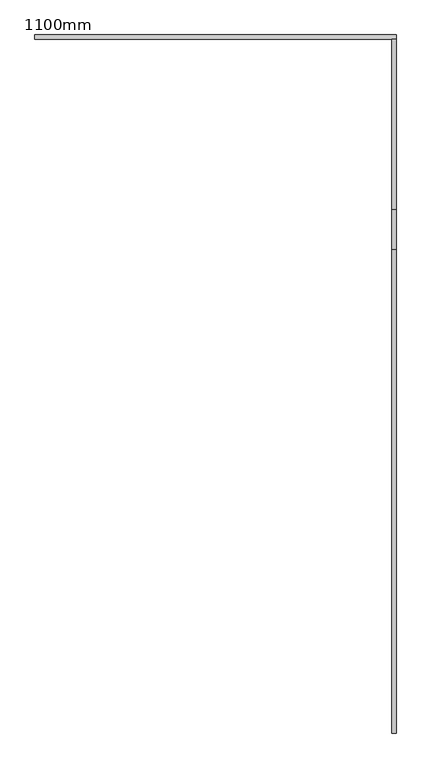
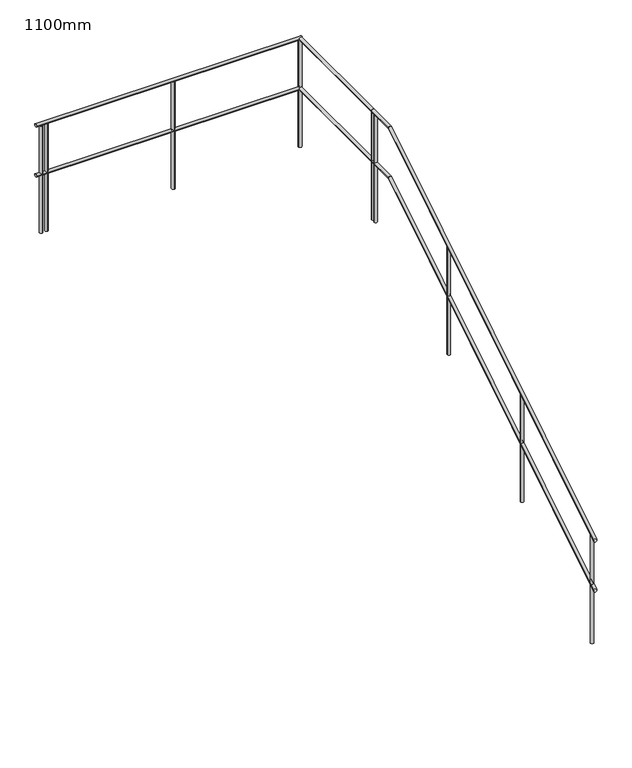
"""IFC4 building model written with IfcOpenShell, lengths in millimetres: railing geometry, 1100mm."""

import ifcopenshell
import ifcopenshell.guid

model = None  # the IFC model being written
_history = None  # IfcOwnerHistory: only IFC2X3 demands one
_inside = {}  # id of a spatial element -> (the spatial element, [elements in it])
_under = {}  # id of a project, library or spatial element -> (it, [spatial elements below it])
_declared = {}  # id of a project -> (the project, [libraries it declares])
_typed = {}  # id of a type object -> (the type object, [elements of that type])
_made_of = {}  # id of a material, layer set ... -> (it, [elements and type objects made of it])


def new_model(schema):
    """Start an empty IFC model of exactly this schema.

    Asked for "IFC4X3", IfcOpenShell would pick the latest addendum, in which some entities
    have other attributes; the version numbers below select the first issue.
    IFC2X3 requires an IfcOwnerHistory on every rooted entity: one is made here for all.
    """
    global model, _history
    if schema == "IFC4X3":
        model = ifcopenshell.file(schema_version=(4, 3, 0, 0))
    else:
        model = ifcopenshell.file(schema=schema)
    _inside.clear()
    _under.clear()
    _declared.clear()
    _typed.clear()
    _made_of.clear()
    _history = None
    if model.schema == "IFC2X3":
        org = make("IfcOrganization", Name="unknown")
        user = make(
            "IfcPersonAndOrganization",
            ThePerson=make("IfcPerson", FamilyName="unknown"),
            TheOrganization=org,
        )
        app = make(
            "IfcApplication",
            ApplicationDeveloper=org,
            Version="unknown",
            ApplicationFullName="unknown",
            ApplicationIdentifier="unknown",
        )
        _history = make(
            "IfcOwnerHistory",
            OwningUser=user,
            OwningApplication=app,
            ChangeAction="ADDED",
            CreationDate=0,
        )
    return model


def make(cls, **values):
    """One entity of the class cls with the attributes given. An attribute that is None is left unset."""
    return model.create_entity(
        cls, **{name: value for name, value in values.items() if value is not None}
    )


def rooted(cls, **values):
    """An entity with a GlobalId (a new one), such as an element, a storey or a relation."""
    return make(cls, GlobalId=ifcopenshell.guid.new(), OwnerHistory=_history, **values)


def si_unit(unit_type, name, prefix=None):
    """IfcSIUnit, for example si_unit("LENGTHUNIT", "METRE", prefix="MILLI")."""
    return make("IfcSIUnit", UnitType=unit_type, Prefix=prefix, Name=name)


def assignment(units):
    """IfcUnitAssignment: the units of a project."""
    return None if units is None else make("IfcUnitAssignment", Units=units)


def point(xyz):
    """IfcCartesianPoint."""
    return None if xyz is None else make("IfcCartesianPoint", Coordinates=xyz)


def direction(xyz):
    """IfcDirection."""
    return None if xyz is None else make("IfcDirection", DirectionRatios=xyz)


def frame(location, z_axis=None, x_axis=None):
    """IfcAxis2Placement3D, a coordinate frame: its origin and axes. An axis left out is left unset."""
    return make(
        "IfcAxis2Placement3D",
        Location=point(location),
        Axis=direction(z_axis),
        RefDirection=direction(x_axis),
    )


def frame_2d(location, x_axis=None):
    """IfcAxis2Placement2D, a coordinate frame in the plane: its origin and x axis."""
    return make(
        "IfcAxis2Placement2D", Location=point(location), RefDirection=direction(x_axis)
    )


def origin():
    """The frame at (0, 0, 0) with its axes left unset."""
    return frame((0.0, 0.0, 0.0))


def place(relative_to, where):
    """IfcLocalPlacement: puts the frame where relative to a parent placement (None: the world)."""
    return make(
        "IfcLocalPlacement", PlacementRelTo=relative_to, RelativePlacement=where
    )


def context(
    kind, dimensions, precision=None, world=None, true_north=None, identifier=None
):
    """IfcGeometricRepresentationContext, for example the 3D "Model" context."""
    return make(
        "IfcGeometricRepresentationContext",
        ContextIdentifier=identifier,
        ContextType=kind,
        CoordinateSpaceDimension=dimensions,
        Precision=precision,
        WorldCoordinateSystem=world,
        TrueNorth=true_north,
    )


def project(units=None, contexts=None):
    """IfcProject with its units and contexts."""
    return rooted(
        "IfcProject",
        Name="project",
        RepresentationContexts=contexts,
        UnitsInContext=assignment(units),
    )


def spatial(cls, under=None, at=None, **own):
    """A site, building, storey or space (cls), placed at a placement, below another one or the project."""
    s = rooted(cls, ObjectPlacement=at, **own)
    if under is not None:
        _under.setdefault(under.id(), (under, []))[1].append(s)
    return s


def circle_curve(where, radius):
    """IfcCircle in the frame where."""
    return make("IfcCircle", Position=where, Radius=radius)


def ellipse_curve(where, semi_axis1, semi_axis2):
    """IfcEllipse in the frame where."""
    return make(
        "IfcEllipse", Position=where, SemiAxis1=semi_axis1, SemiAxis2=semi_axis2
    )


def trimmed(basis, trim1, trim2, sense, master):
    """IfcTrimmedCurve: the piece of a basis curve between two trims."""
    return make(
        "IfcTrimmedCurve",
        BasisCurve=basis,
        Trim1=trim1,
        Trim2=trim2,
        SenseAgreement=sense,
        MasterRepresentation=master,
    )


def segment(curve, same_sense, transition):
    """IfcCompositeCurveSegment."""
    return make(
        "IfcCompositeCurveSegment",
        Transition=transition,
        SameSense=same_sense,
        ParentCurve=curve,
    )


def composite_curve(segments, self_intersect=None):
    """IfcCompositeCurve: segments joined end to end."""
    return make("IfcCompositeCurve", Segments=segments, SelfIntersect=self_intersect)


def outline(outer, holes=None, kind="AREA"):
    """IfcArbitraryClosedProfileDef: a profile drawn as a closed curve; with holes, ...WithVoids."""
    if holes is None:
        return make("IfcArbitraryClosedProfileDef", ProfileType=kind, OuterCurve=outer)
    return make(
        "IfcArbitraryProfileDefWithVoids",
        ProfileType=kind,
        OuterCurve=outer,
        InnerCurves=holes,
    )


def extrude(swept, where, along, depth):
    """IfcExtrudedAreaSolid: the profile swept, set in the frame where, extruded along a direction by depth."""
    return make(
        "IfcExtrudedAreaSolid",
        SweptArea=swept,
        Position=where,
        ExtrudedDirection=direction(along),
        Depth=depth,
    )


def shape(context_of_items, identifier, shape_type, items):
    """IfcShapeRepresentation: the items that make up one representation, for example the "Body"."""
    return make(
        "IfcShapeRepresentation",
        ContextOfItems=context_of_items,
        RepresentationIdentifier=identifier,
        RepresentationType=shape_type,
        Items=items,
    )


def source(mapping_origin, context_of_items, identifier, shape_type, items):
    """IfcRepresentationMap: a shape defined once, which mapped items show again and again."""
    return make(
        "IfcRepresentationMap",
        MappingOrigin=mapping_origin,
        MappedRepresentation=shape(context_of_items, identifier, shape_type, items),
    )


def transform(
    local_origin,
    x_axis=None,
    y_axis=None,
    z_axis=None,
    scale=None,
    scale2=None,
    scale3=None,
    uniform=True,
):
    """IfcCartesianTransformationOperator3D, or its non-uniform kind. x_axis, y_axis, z_axis: its Axis1, 2, 3."""
    if uniform:
        return make(
            "IfcCartesianTransformationOperator3D",
            Axis1=direction(x_axis),
            Axis2=direction(y_axis),
            LocalOrigin=point(local_origin),
            Scale=scale,
            Axis3=direction(z_axis),
        )
    return make(
        "IfcCartesianTransformationOperator3DnonUniform",
        Axis1=direction(x_axis),
        Axis2=direction(y_axis),
        LocalOrigin=point(local_origin),
        Scale=scale,
        Axis3=direction(z_axis),
        Scale2=scale2,
        Scale3=scale3,
    )


def mapped(mapping_source, mapping_target):
    """IfcMappedItem: shows the shape of a source again, moved by a transform."""
    return make(
        "IfcMappedItem", MappingSource=mapping_source, MappingTarget=mapping_target
    )


def made_of(thing, what):
    """Note that an element or type object is made of a material, layer set ...; save() writes the relation."""
    if what is not None:
        _made_of.setdefault(what.id(), (what, []))[1].append(thing)
    return thing


def element(
    cls,
    number,
    at=None,
    inside=None,
    cuts=None,
    type_object=None,
    material=None,
    context=None,
    identifier="Body",
    shape_type=None,
    held_by="IfcProductDefinitionShape",
    body=None,
    shapes=None,
    **own,
):
    """One element of the class cls, such as IfcWall. Its Tag is "e" and its number.

    at: its placement. inside: the storey or other place that contains it. cuts: it is an
    opening in that element (IfcRelVoidsElement). A single representation is given by context,
    identifier, shape_type and body (its items); several are given by shapes. held_by: the class
    of the entity that holds the representations. save() writes the other relations.
    """
    e = rooted(cls, Tag="e%d" % number, ObjectPlacement=at, **own)
    if body is not None:
        shapes = [shape(context, identifier, shape_type, body)]
    if shapes is not None:
        e.Representation = make(held_by, Representations=shapes)
    if inside is not None:
        _inside.setdefault(inside.id(), (inside, []))[1].append(e)
    if cuts is not None:
        rooted(
            "IfcRelVoidsElement", RelatingBuildingElement=cuts, RelatedOpeningElement=e
        )
    if type_object is not None:
        _typed.setdefault(type_object.id(), (type_object, []))[1].append(e)
    return made_of(e, material)


def aggregate(whole, parts):
    """IfcRelAggregates: a whole, such as a stair, and the parts it consists of."""
    return rooted("IfcRelAggregates", RelatingObject=whole, RelatedObjects=parts)


def save(model, path):
    """Write the relations noted so far, then the file.

    IfcRelAggregates (storeys below a building ...), IfcRelContainedInSpatialStructure (elements
    in a storey), IfcRelDefinesByType, IfcRelAssociatesMaterial and IfcRelDeclares: one each for
    every whole, place, type object, material and project.
    """
    for whole, parts in _under.values():
        aggregate(whole, parts)
    for where, things in _inside.values():
        rooted(
            "IfcRelContainedInSpatialStructure",
            RelatedElements=things,
            RelatingStructure=where,
        )
    for kind, things in _typed.values():
        rooted("IfcRelDefinesByType", RelatedObjects=things, RelatingType=kind)
    for what, things in _made_of.values():
        rooted("IfcRelAssociatesMaterial", RelatedObjects=things, RelatingMaterial=what)
    for by, libraries in _declared.values():
        rooted("IfcRelDeclares", RelatingContext=by, RelatedDefinitions=libraries)
    model.write(path)


def plane_surface(at):
    """IfcPlane: the flat surface through the origin of the frame at, square to its z axis."""
    return make("IfcPlane", Position=at)


def cylinder_surface(at, radius):
    """IfcCylindricalSurface: all points at the distance radius from the z axis of the frame at."""
    return make("IfcCylindricalSurface", Position=at, Radius=radius)


def advanced_brep(points, edges, surfaces, faces):
    """IfcAdvancedBrep: a solid bounded by faces that lie on surfaces and meet in shared edges.

    An edge is (start, end): straight between two places in points (the first is 0);
    or (start, end, curve); or (start, end, curve, False) where it runs against its curve.
    A face is (place in surfaces, loops), or (place, loops, False) where it looks against
    its surface's normal. A loop lists edges by number (the first is 1), with a minus sign
    where the edge is run from its end to its start. The first loop is the outer one.
    """
    corners = [point(p) for p in points]
    vertices = [make("IfcVertexPoint", VertexGeometry=c) for c in corners]
    made = []
    for start, end, *more in edges:
        made.append(
            make(
                "IfcEdgeCurve",
                EdgeStart=vertices[start],
                EdgeEnd=vertices[end],
                EdgeGeometry=more[0] if more else make("IfcPolyline", Points=[corners[start], corners[end]]),
                SameSense=more[1] if len(more) > 1 else True,
            )
        )
    hull = []
    for where, loops, *sense in faces:
        bounds = []
        for j, loop in enumerate(loops):
            ring = [make("IfcOrientedEdge", EdgeElement=made[abs(k) - 1], Orientation=k > 0) for k in loop]
            bounds.append(
                make(
                    "IfcFaceOuterBound" if j == 0 else "IfcFaceBound",
                    Bound=make("IfcEdgeLoop", EdgeList=ring),
                    Orientation=True,
                )
            )
        hull.append(make("IfcAdvancedFace", Bounds=bounds, FaceSurface=surfaces[where], SameSense=sense[0] if sense else True))
    return make("IfcAdvancedBrep", Outer=make("IfcClosedShell", CfsFaces=hull))


def railing_1100mm_b1036d3c(model_context):
    return source(origin(), model_context, "Body", "SolidModel", [
        advanced_brep(
        [(12740.5052251, 14699.5208589, 456.3396197), (12710.5052251, 14699.5208589, 456.3396197), (12740.5052251, 18339.5208589, 2547.0), (12710.5052251, 18339.5208589, 2547.0), (12740.5052251, 18063.8019306, 2547.0), (12710.5052251, 18063.8019306, 2547.0)],
        [
            (0, 1, ellipse_curve(frame((12725.5052251, 14699.5208589, 456.3396197), z_axis=(0.0, -1.0, 0.0), x_axis=(0.0, 0.0, -1.0)), 17.6603803, 15.0)),
            (1, 0, ellipse_curve(frame((12725.5052251, 14699.5208589, 456.3396197), z_axis=(0.0, -1.0, 0.0), x_axis=(0.0, 0.0, -1.0)), 17.6603803, 15.0)),
            (2, 3, circle_curve(frame((12725.5052251, 18339.5208589, 2547.0), z_axis=(0.0, 1.0, 0.0), x_axis=(-1.0, 0.0, 0.0)), 15.0)),
            (3, 2, circle_curve(frame((12725.5052251, 18339.5208589, 2547.0), z_axis=(0.0, 1.0, 0.0), x_axis=(-1.0, 0.0, 0.0)), 15.0)),
            (0, 4),
            (4, 5, ellipse_curve(frame((12725.5052251, 18063.8019306, 2547.0), z_axis=(0.0, -0.9616025257983003, -0.2744459552959912), x_axis=(0.0, 0.2744459552959914, -0.9616025257983002)), 15.5989607, 15.0)),
            (5, 1),
            (5, 4, ellipse_curve(frame((12725.5052251, 18063.8019306, 2547.0), z_axis=(0.0, -0.9616025257983003, -0.2744459552959912), x_axis=(0.0, 0.2744459552959914, -0.9616025257983002)), 15.5989607, 15.0)),
            (4, 2),
            (3, 5),
        ],
        [
            plane_surface(frame((12725.5052251, 14699.5208589, 474.0), z_axis=(0.0, -1.0, 0.0), x_axis=(0.0, 0.0, 1.0))),
            plane_surface(frame((12725.5052251, 18339.5208589, 2562.0), z_axis=(0.0, 1.0, 0.0), x_axis=(0.0, 0.0, 1.0))),
            cylinder_surface(frame((12725.5052251, 14707.4380966, 461.2596175), z_axis=(0.0, -0.8493588352433417, -0.5278158476155052), x_axis=(-1.0, 0.0, 0.0)), 15.0),
            cylinder_surface(frame((12725.5052251, 18059.5208589, 2547.0), z_axis=(0.0, -1.0, 0.0), x_axis=(-1.0, 0.0, 0.0)), 15.0),
        ],
        [
            (0, [[1, 2]]),
            (1, [[3, 4]]),
            (2, [[-1, 5, 6, 7]]),
            (2, [[-2, -7, 8, -5]]),
            (3, [[-6, 9, -4, 10]]),
            (3, [[-8, -10, -3, -9]]),
        ],
    ),
        advanced_brep(
        [(12740.5052251, 18339.5208589, 2547.0), (12710.5052251, 18339.5208589, 2547.0), (12740.5052251, 19524.9208589, 2547.0), (12710.5052251, 19524.9208589, 2547.0)],
        [
            (0, 1, circle_curve(frame((12725.5052251, 18339.5208589, 2547.0), z_axis=(0.0, -1.0, 0.0), x_axis=(-1.0, 0.0, 0.0)), 15.0)),
            (1, 0, circle_curve(frame((12725.5052251, 18339.5208589, 2547.0), z_axis=(0.0, -1.0, 0.0), x_axis=(-1.0, 0.0, 0.0)), 15.0)),
            (2, 3, circle_curve(frame((12725.5052251, 19524.9208589, 2547.0), z_axis=(0.0, 1.0, 0.0), x_axis=(-1.0, 0.0, 0.0)), 15.0)),
            (3, 2, circle_curve(frame((12725.5052251, 19524.9208589, 2547.0), z_axis=(0.0, 1.0, 0.0), x_axis=(-1.0, 0.0, 0.0)), 15.0)),
            (0, 2),
            (3, 1),
        ],
        [
            plane_surface(frame((12725.5052251, 18339.5208589, 2562.0), z_axis=(0.0, -1.0, 0.0), x_axis=(0.0, 0.0, 1.0))),
            plane_surface(frame((12725.5052251, 19524.9208589, 2562.0), z_axis=(0.0, 1.0, 0.0), x_axis=(0.0, 0.0, 1.0))),
            cylinder_surface(frame((12725.5052251, 18339.5208589, 2547.0), z_axis=(0.0, -1.0, 0.0), x_axis=(-1.0, 0.0, 0.0)), 15.0),
        ],
        [
            (0, [[1, 2]]),
            (1, [[3, 4]]),
            (2, [[-1, 5, -4, 6]]),
            (2, [[-2, -6, -3, -5]]),
        ],
    ),
        advanced_brep(
        [(12740.5052251, 19554.9208589, 2547.0), (12740.5052251, 19524.9208589, 2547.0), (10225.1052251, 19554.9208589, 2547.0), (10225.1052251, 19524.9208589, 2547.0)],
        [
            (0, 1, circle_curve(frame((12740.5052251, 19539.9208589, 2547.0), z_axis=(1.0, 0.0, 0.0), x_axis=(0.0, -1.0, 0.0)), 15.0)),
            (1, 0, circle_curve(frame((12740.5052251, 19539.9208589, 2547.0), z_axis=(1.0, 0.0, 0.0), x_axis=(0.0, -1.0, 0.0)), 15.0)),
            (2, 3, circle_curve(frame((10225.1052251, 19539.9208589, 2547.0), z_axis=(-1.0, 0.0, 0.0), x_axis=(0.0, -1.0, 0.0)), 15.0)),
            (3, 2, circle_curve(frame((10225.1052251, 19539.9208589, 2547.0), z_axis=(-1.0, 0.0, 0.0), x_axis=(0.0, -1.0, 0.0)), 15.0)),
            (0, 2),
            (3, 1),
        ],
        [
            plane_surface(frame((12740.5052251, 19539.9208589, 2562.0), z_axis=(1.0, 0.0, 0.0), x_axis=(0.0, -1.0, 0.0))),
            plane_surface(frame((10225.1052251, 19539.9208589, 2562.0), z_axis=(-1.0, 0.0, 0.0), x_axis=(0.0, -1.0, 0.0))),
            cylinder_surface(frame((12740.5052251, 19539.9208589, 2547.0), z_axis=(1.0, 0.0, 0.0), x_axis=(0.0, -1.0, 0.0)), 15.0),
        ],
        [
            (0, [[1, 2]]),
            (1, [[3, 4]]),
            (2, [[-1, 5, -4, 6]]),
            (2, [[-2, -6, -3, -5]]),
        ],
    ),
        advanced_brep(
        [(12740.5052251, 14699.5208589, 956.3396197), (12710.5052251, 14699.5208589, 956.3396197), (12740.5052251, 18063.8019306, 3047.0), (12710.5052251, 18063.8019306, 3047.0), (12740.5052251, 18339.5208589, 3047.0), (12710.5052251, 18339.5208589, 3047.0)],
        [
            (0, 1, ellipse_curve(frame((12725.5052251, 14699.5208589, 956.3396197), z_axis=(0.0, -1.0, 0.0), x_axis=(0.0, 0.0, -1.0)), 17.6603803, 15.0)),
            (1, 0, ellipse_curve(frame((12725.5052251, 14699.5208589, 956.3396197), z_axis=(0.0, -1.0, 0.0), x_axis=(0.0, 0.0, -1.0)), 17.6603803, 15.0)),
            (0, 2),
            (2, 3, ellipse_curve(frame((12725.5052251, 18063.8019306, 3047.0), z_axis=(0.0, -0.9616025257983003, -0.2744459552959912), x_axis=(0.0, 0.2744459552959914, -0.9616025257983002)), 15.5989607, 15.0)),
            (3, 1),
            (3, 2, ellipse_curve(frame((12725.5052251, 18063.8019306, 3047.0), z_axis=(0.0, -0.9616025257983003, -0.2744459552959912), x_axis=(0.0, 0.2744459552959914, -0.9616025257983002)), 15.5989607, 15.0)),
            (4, 5, circle_curve(frame((12725.5052251, 18339.5208589, 3047.0), z_axis=(0.0, 1.0, 0.0), x_axis=(-1.0, 0.0, 0.0)), 15.0)),
            (5, 4, circle_curve(frame((12725.5052251, 18339.5208589, 3047.0), z_axis=(0.0, 1.0, 0.0), x_axis=(-1.0, 0.0, 0.0)), 15.0)),
            (2, 4),
            (5, 3),
        ],
        [
            plane_surface(frame((12725.5052251, 14699.5208589, 974.0), z_axis=(0.0, -1.0, 0.0), x_axis=(0.0, 0.0, 1.0))),
            cylinder_surface(frame((12725.5052251, 14707.4380966, 961.2596175), z_axis=(0.0, -0.8493588352433417, -0.5278158476155052), x_axis=(-1.0, 0.0, 0.0)), 15.0),
            plane_surface(frame((12725.5052251, 18339.5208589, 3062.0), z_axis=(0.0, 1.0, 0.0), x_axis=(0.0, 0.0, 1.0))),
            cylinder_surface(frame((12725.5052251, 18059.5208589, 3047.0), z_axis=(0.0, -1.0, 0.0), x_axis=(-1.0, 0.0, 0.0)), 15.0),
        ],
        [
            (0, [[1, 2]]),
            (1, [[-1, 3, 4, 5]]),
            (1, [[-2, -5, 6, -3]]),
            (2, [[7, 8]]),
            (3, [[-4, 9, -8, 10]]),
            (3, [[-6, -10, -7, -9]]),
        ],
    ),
        advanced_brep(
        [(12740.5052251, 18339.5208589, 3047.0), (12710.5052251, 18339.5208589, 3047.0), (12740.5052251, 19524.9208589, 3047.0), (12710.5052251, 19524.9208589, 3047.0)],
        [
            (0, 1, circle_curve(frame((12725.5052251, 18339.5208589, 3047.0), z_axis=(0.0, -1.0, 0.0), x_axis=(-1.0, 0.0, 0.0)), 15.0)),
            (1, 0, circle_curve(frame((12725.5052251, 18339.5208589, 3047.0), z_axis=(0.0, -1.0, 0.0), x_axis=(-1.0, 0.0, 0.0)), 15.0)),
            (2, 3, circle_curve(frame((12725.5052251, 19524.9208589, 3047.0), z_axis=(0.0, 1.0, 0.0), x_axis=(-1.0, 0.0, 0.0)), 15.0)),
            (3, 2, circle_curve(frame((12725.5052251, 19524.9208589, 3047.0), z_axis=(0.0, 1.0, 0.0), x_axis=(-1.0, 0.0, 0.0)), 15.0)),
            (0, 2),
            (3, 1),
        ],
        [
            plane_surface(frame((12725.5052251, 18339.5208589, 3062.0), z_axis=(0.0, -1.0, 0.0), x_axis=(0.0, 0.0, 1.0))),
            plane_surface(frame((12725.5052251, 19524.9208589, 3062.0), z_axis=(0.0, 1.0, 0.0), x_axis=(0.0, 0.0, 1.0))),
            cylinder_surface(frame((12725.5052251, 18339.5208589, 3047.0), z_axis=(0.0, -1.0, 0.0), x_axis=(-1.0, 0.0, 0.0)), 15.0),
        ],
        [
            (0, [[1, 2]]),
            (1, [[3, 4]]),
            (2, [[-1, 5, -4, 6]]),
            (2, [[-2, -6, -3, -5]]),
        ],
    ),
        advanced_brep(
        [(12740.5052251, 19554.9208589, 3047.0), (12740.5052251, 19524.9208589, 3047.0), (10225.1052251, 19554.9208589, 3047.0), (10225.1052251, 19524.9208589, 3047.0)],
        [
            (0, 1, circle_curve(frame((12740.5052251, 19539.9208589, 3047.0), z_axis=(1.0, 0.0, 0.0), x_axis=(0.0, -1.0, 0.0)), 15.0)),
            (1, 0, circle_curve(frame((12740.5052251, 19539.9208589, 3047.0), z_axis=(1.0, 0.0, 0.0), x_axis=(0.0, -1.0, 0.0)), 15.0)),
            (2, 3, circle_curve(frame((10225.1052251, 19539.9208589, 3047.0), z_axis=(-1.0, 0.0, 0.0), x_axis=(0.0, -1.0, 0.0)), 15.0)),
            (3, 2, circle_curve(frame((10225.1052251, 19539.9208589, 3047.0), z_axis=(-1.0, 0.0, 0.0), x_axis=(0.0, -1.0, 0.0)), 15.0)),
            (0, 2),
            (3, 1),
        ],
        [
            plane_surface(frame((12740.5052251, 19539.9208589, 3062.0), z_axis=(1.0, 0.0, 0.0), x_axis=(0.0, -1.0, 0.0))),
            plane_surface(frame((10225.1052251, 19539.9208589, 3062.0), z_axis=(-1.0, 0.0, 0.0), x_axis=(0.0, -1.0, 0.0))),
            cylinder_surface(frame((12740.5052251, 19539.9208589, 3047.0), z_axis=(1.0, 0.0, 0.0), x_axis=(0.0, -1.0, 0.0)), 15.0),
        ],
        [
            (0, [[1, 2]]),
            (1, [[3, 4]]),
            (2, [[-1, 5, -4, 6]]),
            (2, [[-2, -6, -3, -5]]),
        ],
    ),
        extrude(outline(composite_curve([segment(trimmed(circle_curve(frame_2d((10325.5052251, 19539.9208589)), 15.0), [point((10325.5052251, 19524.9208589))], [point((10325.5052251, 19554.9208589))], False, "CARTESIAN"), True, "CONTINUOUS"), segment(trimmed(circle_curve(frame_2d((10325.5052251, 19539.9208589)), 15.0), [point((10325.5052251, 19554.9208589))], [point((10325.5052251, 19524.9208589))], False, "CARTESIAN"), True, "CONTINUOUS")], self_intersect=False)), frame((0.0, 0.0, 1962.0), z_axis=(0.0, 0.0, 1.0), x_axis=(1.0, 0.0, 0.0)), (0.0, 0.0, 1.0), 1070.0),
        extrude(outline(composite_curve([segment(trimmed(circle_curve(frame_2d((11525.5052251, 19539.9208589)), 15.0), [point((11525.5052251, 19524.9208589))], [point((11525.5052251, 19554.9208589))], False, "CARTESIAN"), True, "CONTINUOUS"), segment(trimmed(circle_curve(frame_2d((11525.5052251, 19539.9208589)), 15.0), [point((11525.5052251, 19554.9208589))], [point((11525.5052251, 19524.9208589))], False, "CARTESIAN"), True, "CONTINUOUS")], self_intersect=False)), frame((0.0, 0.0, 1962.0), z_axis=(0.0, 0.0, 1.0), x_axis=(1.0, 0.0, 0.0)), (0.0, 0.0, 1.0), 1070.0),
        extrude(outline(composite_curve([segment(trimmed(circle_curve(frame_2d((12725.5052251, 19539.5208589)), 15.0), [point((12710.5052251, 19539.5208589))], [point((12740.5052251, 19539.5208589))], False, "CARTESIAN"), True, "CONTINUOUS"), segment(trimmed(circle_curve(frame_2d((12725.5052251, 19539.5208589)), 15.0), [point((12740.5052251, 19539.5208589))], [point((12710.5052251, 19539.5208589))], False, "CARTESIAN"), True, "CONTINUOUS")], self_intersect=False)), frame((0.0, 0.0, 1962.0), z_axis=(0.0, 0.0, 1.0), x_axis=(1.0, 0.0, 0.0)), (0.0, 0.0, 1.0), 1070.0),
        extrude(outline(composite_curve([segment(trimmed(circle_curve(frame_2d((12725.5052251, 18299.5208589)), 15.0), [point((12710.5052251, 18299.5208589))], [point((12740.5052251, 18299.5208589))], False, "CARTESIAN"), True, "CONTINUOUS"), segment(trimmed(circle_curve(frame_2d((12725.5052251, 18299.5208589)), 15.0), [point((12740.5052251, 18299.5208589))], [point((12710.5052251, 18299.5208589))], False, "CARTESIAN"), True, "CONTINUOUS")], self_intersect=False)), frame((0.0, 0.0, 1962.0), z_axis=(0.0, 0.0, 1.0), x_axis=(1.0, 0.0, 0.0)), (0.0, 0.0, 1.0), 1070.0),
        extrude(outline(composite_curve([segment(trimmed(circle_curve(frame_2d((12725.5052251, 17099.5208589)), 15.0), [point((12710.5052251, 17099.5208589))], [point((12740.5052251, 17099.5208589))], False, "CARTESIAN"), True, "CONTINUOUS"), segment(trimmed(circle_curve(frame_2d((12725.5052251, 17099.5208589)), 15.0), [point((12740.5052251, 17099.5208589))], [point((12710.5052251, 17099.5208589))], False, "CARTESIAN"), True, "CONTINUOUS")], self_intersect=False)), frame((0.0, 0.0, 1365.4285714), z_axis=(0.0, 0.0, 1.0), x_axis=(1.0, 0.0, 0.0)), (0.0, 0.0, 1.0), 1070.0),
        extrude(outline(composite_curve([segment(trimmed(circle_curve(frame_2d((12725.5052251, 15899.5208589)), 15.0), [point((12710.5052251, 15899.5208589))], [point((12740.5052251, 15899.5208589))], False, "CARTESIAN"), True, "CONTINUOUS"), segment(trimmed(circle_curve(frame_2d((12725.5052251, 15899.5208589)), 15.0), [point((12740.5052251, 15899.5208589))], [point((12710.5052251, 15899.5208589))], False, "CARTESIAN"), True, "CONTINUOUS")], self_intersect=False)), frame((0.0, 0.0, 619.7142857), z_axis=(0.0, 0.0, 1.0), x_axis=(1.0, 0.0, 0.0)), (0.0, 0.0, 1.0), 1070.0),
        extrude(outline(composite_curve([segment(trimmed(circle_curve(frame_2d((12725.5052251, 19539.9208589)), 15.0), [point((12710.5052251, 19539.9208589))], [point((12740.5052251, 19539.9208589))], False, "CARTESIAN"), True, "CONTINUOUS"), segment(trimmed(circle_curve(frame_2d((12725.5052251, 19539.9208589)), 15.0), [point((12740.5052251, 19539.9208589))], [point((12710.5052251, 19539.9208589))], False, "CARTESIAN"), True, "CONTINUOUS")], self_intersect=False)), frame((0.0, 0.0, 1962.0), z_axis=(0.0, 0.0, 1.0), x_axis=(1.0, 0.0, 0.0)), (0.0, 0.0, 1.0), 1070.0),
        extrude(outline(composite_curve([segment(trimmed(circle_curve(frame_2d((12725.5052251, 18339.5208589)), 15.0), [point((12710.5052251, 18339.5208589))], [point((12740.5052251, 18339.5208589))], False, "CARTESIAN"), True, "CONTINUOUS"), segment(trimmed(circle_curve(frame_2d((12725.5052251, 18339.5208589)), 15.0), [point((12740.5052251, 18339.5208589))], [point((12710.5052251, 18339.5208589))], False, "CARTESIAN"), True, "CONTINUOUS")], self_intersect=False)), frame((0.0, 0.0, 1962.0), z_axis=(0.0, 0.0, 1.0), x_axis=(1.0, 0.0, 0.0)), (0.0, 0.0, 1.0), 1070.0),
        extrude(outline(composite_curve([segment(trimmed(circle_curve(frame_2d((10275.1052251, 19539.9208589)), 15.0), [point((10275.1052251, 19524.9208589))], [point((10275.1052251, 19554.9208589))], False, "CARTESIAN"), True, "CONTINUOUS"), segment(trimmed(circle_curve(frame_2d((10275.1052251, 19539.9208589)), 15.0), [point((10275.1052251, 19554.9208589))], [point((10275.1052251, 19524.9208589))], False, "CARTESIAN"), True, "CONTINUOUS")], self_intersect=False)), frame((0.0, 0.0, 1962.0), z_axis=(0.0, 0.0, 1.0), x_axis=(1.0, 0.0, 0.0)), (0.0, 0.0, 1.0), 1070.0),
        extrude(outline(composite_curve([segment(trimmed(circle_curve(frame_2d((12725.5052251, 14749.5208589)), 15.0), [point((12710.5052251, 14749.5208589))], [point((12740.5052251, 14749.5208589))], False, "CARTESIAN"), True, "CONTINUOUS"), segment(trimmed(circle_curve(frame_2d((12725.5052251, 14749.5208589)), 15.0), [point((12740.5052251, 14749.5208589))], [point((12710.5052251, 14749.5208589))], False, "CARTESIAN"), True, "CONTINUOUS")], self_intersect=False)), frame((0.0, 0.0, -94.9285714), z_axis=(0.0, 0.0, 1.0), x_axis=(1.0, 0.0, 0.0)), (0.0, 0.0, 1.0), 1070.0),
    ])


if __name__ == "__main__":
    model = new_model("IFC4")
    model_context = context("Model", 3, world=origin())
    ifc_project = project(units=[si_unit("LENGTHUNIT", "METRE", prefix="MILLI")], contexts=[model_context])
    site = spatial("IfcSite", under=ifc_project)
    building = spatial("IfcBuilding", under=site)
    placement = place(None, origin())
    railing_1100mm_shape = railing_1100mm_b1036d3c(model_context)
    element("IfcRailing", 1, ObjectType="1100mm", at=placement, inside=building, context=model_context, shape_type="MappedRepresentation", body=[
        mapped(railing_1100mm_shape, transform((0.0, 0.0, 0.0), x_axis=(1.0, 0.0, 0.0), y_axis=(0.0, 1.0, 0.0), z_axis=(0.0, 0.0, 1.0))),
    ])
    save(model, "model.ifc")
